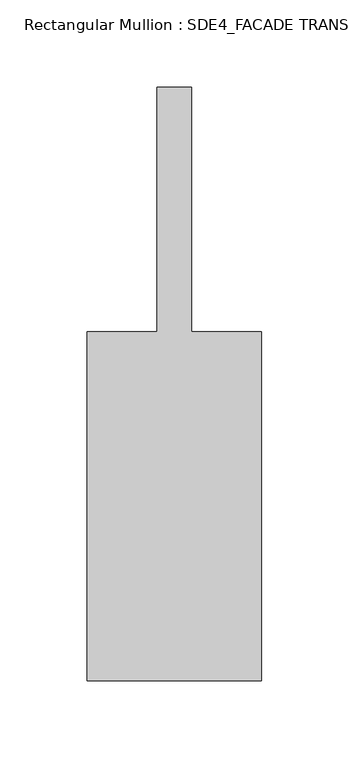
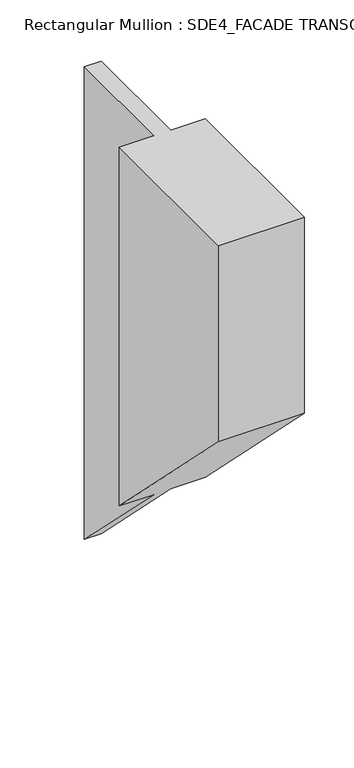
"""IFC4 building model written with IfcOpenShell, lengths in millimetres: member geometry, Rectangular Mullion : SDE4_FACADE TRANSOM TYPE 1."""

from ifc_helpers import new_model, si_unit, origin, place, context, project, spatial, faceted_brep, source, transform, mapped, element, save


def rectangular_mullion_sde4_facade_transom_type_1_3a9d238e(model_context):
    return source(origin(), model_context, "Body", "Brep", [
        faceted_brep([(50.0, -132.5, 0.0), (50.0, 67.5, 0.0), (10.0, 67.5, 0.0), (10.0, 207.5, 0.0), (-10.0, 207.5, 0.0), (-10.0, 67.5, 0.0), (-50.0, 67.5, 0.0), (-50.0, -132.5, 0.0), (50.0, -132.5, -241.2014804), (50.0, 67.5, -441.2014804), (10.0, 67.5, -441.2014804), (10.0, 207.5, -581.2014804), (-10.0, 207.5, -581.2014804), (-10.0, 67.5, -441.2014804), (-50.0, 67.5, -441.2014804), (-50.0, -132.5, -241.2014804)], [[[0, 1, 2, 3, 4, 5, 6, 7]], [[1, 0, 8, 9]], [[2, 1, 9, 10]], [[3, 2, 10, 11]], [[4, 3, 11, 12]], [[5, 4, 12, 13]], [[6, 5, 13, 14]], [[7, 6, 14, 15]], [[0, 7, 15, 8]], [[8, 15, 14, 13, 12, 11, 10, 9]]]),
    ])


if __name__ == "__main__":
    model = new_model("IFC4")
    model_context = context("Model", 3, world=origin())
    ifc_project = project(units=[si_unit("LENGTHUNIT", "METRE", prefix="MILLI")], contexts=[model_context])
    site = spatial("IfcSite", under=ifc_project)
    building = spatial("IfcBuilding", under=site)
    placement = place(None, origin())
    rectangular_mullion_sde4_facade_transom_type_1_shape = rectangular_mullion_sde4_facade_transom_type_1_3a9d238e(model_context)
    element("IfcMember", 1, ObjectType="Rectangular Mullion : SDE4_FACADE TRANSOM TYPE 1", at=placement, inside=building, context=model_context, shape_type="MappedRepresentation", body=[
        mapped(rectangular_mullion_sde4_facade_transom_type_1_shape, transform((0.0, 0.0, 0.0), x_axis=(1.0, 0.0, 0.0), y_axis=(0.0, 1.0, 0.0), z_axis=(0.0, 0.0, 1.0))),
    ])
    save(model, "model.ifc")

# Revit data of these elements
# Type "Rectangular Mullion : SDE4_FACADE TRANSOM TYPE 1"
#   built-in parameter 1007322 = 1.11549 (stored number, unit not read)
#   built-in parameter 1007321 = 0.164042 (stored number, unit not read)
#   built-in parameter 1007320 = 0.164042 (stored number, unit not read)
